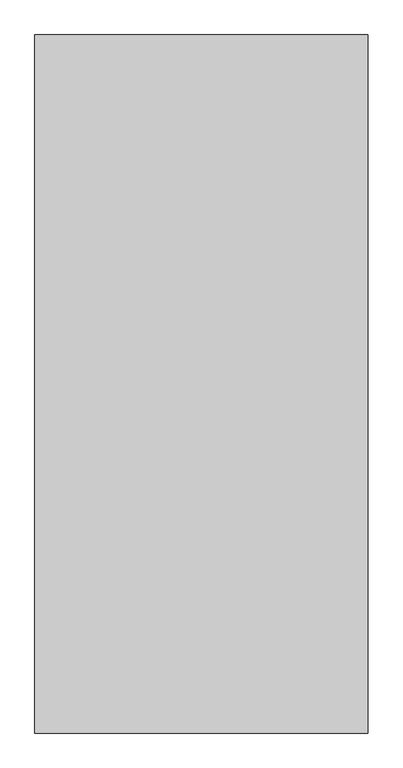
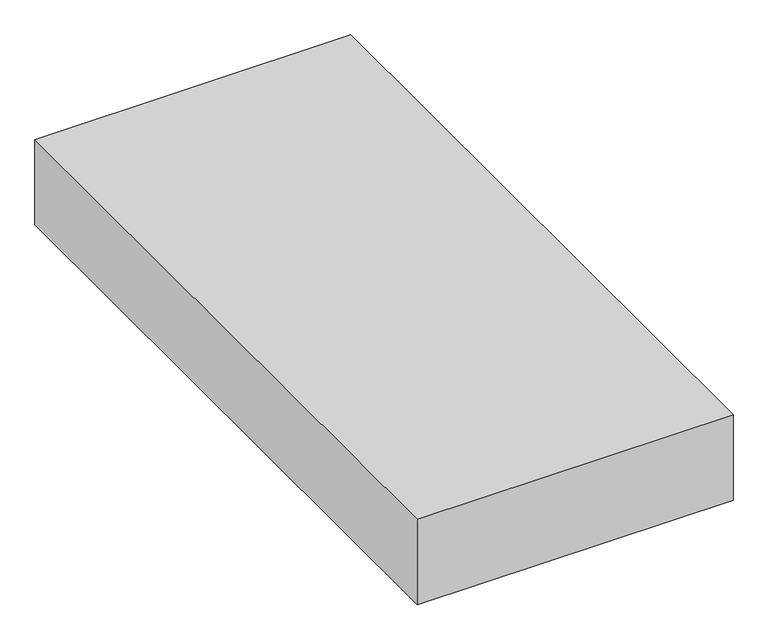
"""IFC4 building model written with IfcOpenShell, lengths in millimetres: proxy geometry, Space Planning Box_hec : Space Planning Box_hec."""

from ifc_helpers import new_model, si_unit, origin, origin_with_axes, place, context, project, spatial, polyline, outline, extrude, source, transform, mapped, element, save


def generic_models_b146db3b(model_context):
    return source(origin(), model_context, "Body", "SweptSolid", [
        extrude(outline(polyline([(10500.0, 22000.0), (10500.0, -22000.0), (-10500.0, -22000.0), (-10500.0, 22000.0), (10500.0, 22000.0)])), origin_with_axes(), (0.0, 0.0, 1.0), 6000.0),
    ])


if __name__ == "__main__":
    model = new_model("IFC4")
    model_context = context("Model", 3, world=origin())
    ifc_project = project(units=[si_unit("LENGTHUNIT", "METRE", prefix="MILLI")], contexts=[model_context])
    site = spatial("IfcSite", under=ifc_project)
    building = spatial("IfcBuilding", under=site)
    placement = place(None, origin())
    generic_models_shape = generic_models_b146db3b(model_context)
    element("IfcBuildingElementProxy", 1, Name="Space Planning Box_hec : Space Planning Box_hec", ObjectType="Space Planning Box_hec : Space Planning Box_hec", at=placement, inside=building, context=model_context, shape_type="MappedRepresentation", body=[
        mapped(generic_models_shape, transform((0.0, 0.0, 0.0), x_axis=(1.0, 0.0, 0.0), y_axis=(0.0, 1.0, 0.0), z_axis=(0.0, 0.0, 1.0))),
    ])
    save(model, "model.ifc")

# Revit data of these elements
# Type "Space Planning Box_hec : Space Planning Box_hec"
#   Type Comments = "..."
#   Room Name [instance default] = "?"
#   Interior Finish [instance default] = ""
#   Exterior Finish [instance default] = ""
#   Department [instance default] = ""
#   Assembly Code = "..."
#   Width [instance default] = 1524 mm
#   Program Area [instance default] = 0.00 m²
#   Length [instance default] = 1524 mm
#   Height [instance default] = 1524 mm
#   Area [instance default] = 2.32258 m²
#   Fill Color [instance default] = Cyan
#   Default Elevation = 0
# Element 1 (IfcBuildingElementProxy, "Space Planning Box_hec : Space Planning Box_hec")
#   Room Name = "Corridor"
#   Interior Finish = "IF2-1"
#   Exterior Finish = "EF1"
#   Department = "AR"
#   Width = 21000 mm
#   Program Area = 86.40 m²
#   Length = 44000 mm
#   Height = 6000 mm
#   Area = 924.00 m²
#   Fill Color = Lavender
#   Materials on its faces: "Lavender"
# Materials
#   "Cyan": class "Generic", colour RGB 0 255 255, transparency 0.2, Cost = 0
#   "Lavender": class "Generic", colour RGB 186 85 211, transparency 0.2, Cost = 0
